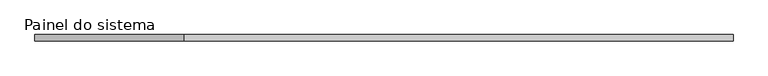
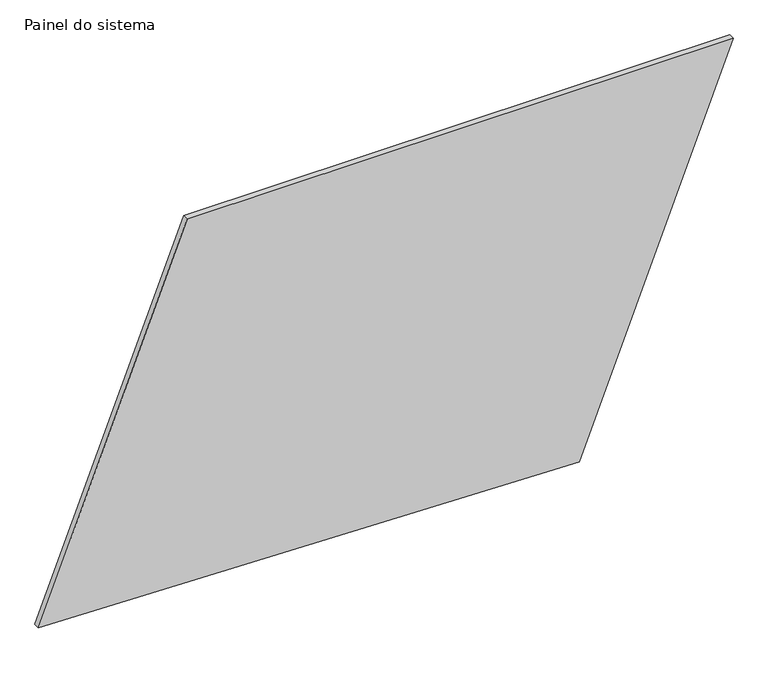
"""IFC4 building model written with IfcOpenShell, lengths in millimetres: plate geometry, Painel do sistema : Envidraçado."""

from ifc_helpers import new_model, si_unit, frame, origin, place, context, project, spatial, polyline, outline, extrude, source, transform, mapped, element, save


def painel_do_sistema_9f8d58e6(model_context):
    return source(origin(), model_context, "Body", "SweptSolid", [
        extrude(outline(polyline([(55.4927774, -1408.0544496), (0.0, 783.8835898), (1597.6714996, 1408.0544496), (1597.6714996, -805.5632496), (55.4927774, -1408.0544496)])), frame((0.0, 24.5, 0.0), z_axis=(0.0, 1.0, 0.0), x_axis=(0.0, 0.0, 1.0)), (0.0, 0.0, 1.0), 25.0),
    ])


if __name__ == "__main__":
    model = new_model("IFC4")
    model_context = context("Model", 3, world=origin())
    ifc_project = project(units=[si_unit("LENGTHUNIT", "METRE", prefix="MILLI")], contexts=[model_context])
    site = spatial("IfcSite", under=ifc_project)
    building = spatial("IfcBuilding", under=site)
    placement = place(None, origin())
    painel_do_sistema_shape = painel_do_sistema_9f8d58e6(model_context)
    element("IfcPlate", 1, ObjectType="Painel do sistema : Envidraçado", at=placement, inside=building, context=model_context, shape_type="MappedRepresentation", body=[
        mapped(painel_do_sistema_shape, transform((0.0, 0.0, 0.0), x_axis=(1.0, 0.0, 0.0), y_axis=(0.0, 1.0, 0.0), z_axis=(0.0, 0.0, 1.0))),
    ])
    save(model, "model.ifc")

# Revit data of these elements
# Type "Painel do sistema : Envidraçado"
#   Construction Type Id = "GSP4R"
#   Analytic Construction = "Vidraça única Pilkington 1/8 pol"
#   Visual Light Transmittance = 0.9
#   Solar Heat Gain Coefficient = 0.86
#   Heat Transfer Coefficient (U) = 6.7069 W/(m²·K)
# Element 1 (IfcPlate, "Painel do sistema : Envidraçado")
#   Materials on its faces: "Vidro"
# Materials
#   "Vidro": class "Vidro", colour RGB 0 128 192, transparency 0.9, Description = "Vidro de sílica", Cost = 0
